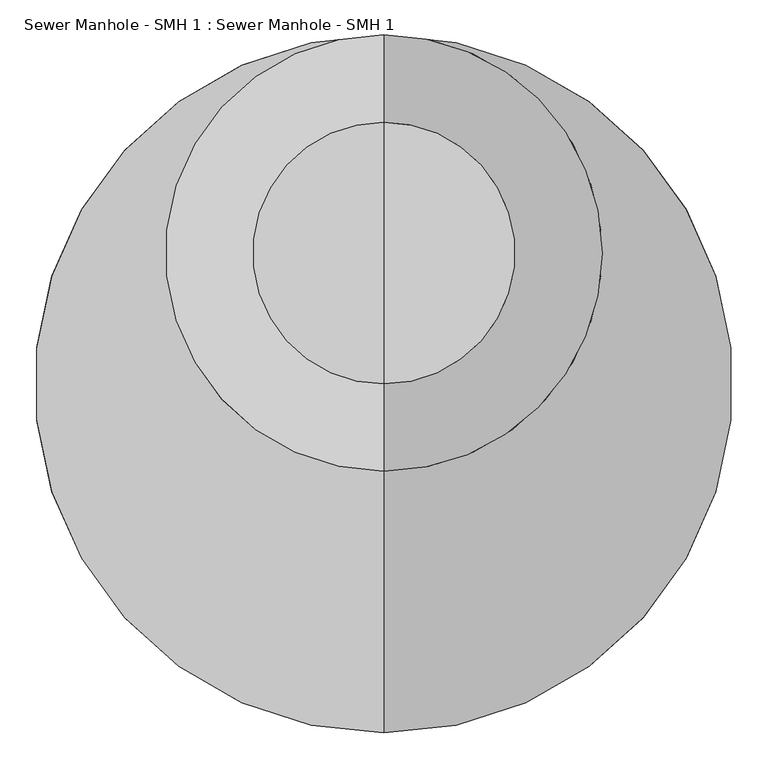
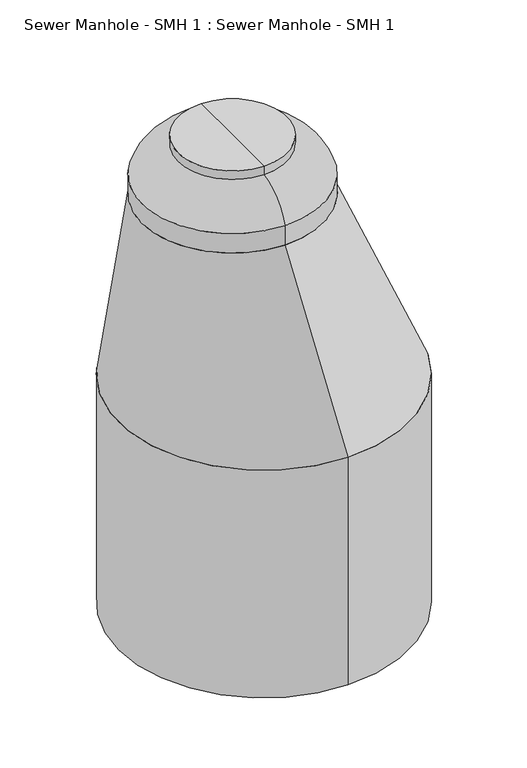
"""IFC4 building model written with IfcOpenShell, lengths in millimetres: proxy geometry, Sewer Manhole - SMH 1 : Sewer Manhole - SMH 1."""

from ifc_helpers import new_model, si_unit, point, frame, origin, place, context, project, spatial, circle_curve, ellipse_curve, trimmed, source, transform, mapped, element, save
from ifc_brep_helpers import plane_surface, cylinder_surface, revolved_surface, spline_surface, advanced_brep


def sewer_manhole_smh_1_sewer_manhole_smh_1_fd977433(model_context):
    return source(origin(), model_context, "Body", "AdvancedBrep", [
        advanced_brep(
        [(0.0, 812.8, 2231.8870774), (0.0, -203.2, 2231.8870774), (0.0, 812.8, 1346.2), (0.0, -812.8, 1346.2)],
        [
            (0, 1, circle_curve(frame((0.0, 304.8, 2231.8870774), z_axis=(0.0, 0.0, 1.0), x_axis=(0.0, 1.0, 0.0)), 508.0)),
            (1, 0, circle_curve(frame((0.0, 304.8, 2231.8870774), z_axis=(0.0, 0.0, 1.0), x_axis=(0.0, 1.0, 0.0)), 508.0)),
            (2, 3, circle_curve(frame((0.0, 0.0, 1346.2), z_axis=(0.0, 0.0, -1.0), x_axis=(0.0, 1.0, 0.0)), 812.8)),
            (3, 2, circle_curve(frame((0.0, 0.0, 1346.2), z_axis=(0.0, 0.0, -1.0), x_axis=(0.0, 1.0, 0.0)), 812.8)),
            (3, 1),
            (0, 2),
        ],
        [
            plane_surface(frame((0.0, 304.8, 2231.8870774), z_axis=(0.0, 0.0, 1.0), x_axis=(1.0, 0.0, 0.0))),
            plane_surface(frame((0.0, 0.0, 1346.2), z_axis=(0.0, 0.0, -1.0), x_axis=(1.0, 0.0, 0.0))),
            spline_surface(2, 1, [[(0.0, 812.8, 1346.2), (0.0, 812.8, 2231.8870774)], [(-812.8, 812.8, 1346.2), (-507.99999999999994, 812.8, 2231.8870774)], [(-812.8, 0.0, 1346.2), (-507.99999999999994, 304.8, 2231.8870774)], [(-812.8, -812.8, 1346.2), (-507.99999999999994, -203.19999999999993, 2231.8870774)], [(0.0, -812.8, 1346.2), (0.0, -203.2, 2231.8870774)]], [3, 2, 3], [2, 2], [0.0, 1.0, 2.0], [0.0, 1.0], weights=[[1.0, 1.0], [0.7071067811865476, 0.7071067811865476], [1.0, 1.0], [0.7071067811865476, 0.7071067811865476], [1.0, 1.0]]),
            spline_surface(2, 1, [[(0.0, -812.8, 1346.2), (0.0, -203.2, 2231.8870774)], [(812.8, -812.8, 1346.2), (508.0, -203.2, 2231.8870774)], [(812.8, 0.0, 1346.2), (508.0, 304.8, 2231.8870774)], [(812.8, 812.8, 1346.2), (508.0, 812.8, 2231.8870774)], [(0.0, 812.8, 1346.2), (0.0, 812.8, 2231.8870774)]], [3, 2, 3], [2, 2], [0.0, 1.0, 2.0], [0.0, 1.0], weights=[[1.0, 1.0], [0.7071067811865476, 0.7071067811865476], [1.0, 1.0], [0.7071067811865476, 0.7071067811865476], [1.0, 1.0]]),
        ],
        [
            (0, [[1, 2]]),
            (1, [[3, 4]]),
            (2, [[-4, 5, -1, 6]]),
            (3, [[-3, -6, -2, -5]]),
        ],
    ),
        advanced_brep(
        [(0.0, -203.2, 2231.8870774), (0.0, 812.8, 2231.8870774), (0.0, 304.8, 2231.8870774), (0.0, -203.2, 2346.96), (0.0, 812.8, 2346.96), (0.0, 0.0, 2524.76), (0.0, 609.6, 2524.76), (0.0, 0.0, 2575.56), (0.0, 609.6, 2575.56), (0.0, 304.8, 2575.56)],
        [
            (0, 1, circle_curve(frame((0.0, 304.8, 2231.8870774), z_axis=(0.0, 0.0, -1.0), x_axis=(0.0, 1.0, 0.0)), 508.0)),
            (1, 2),
            (2, 0),
            (1, 0, circle_curve(frame((0.0, 304.8, 2231.8870774), z_axis=(0.0, 0.0, -1.0), x_axis=(0.0, 1.0, 0.0)), 508.0)),
            (3, 4, circle_curve(frame((0.0, 304.8, 2346.96), z_axis=(0.0, 0.0, -1.0), x_axis=(0.0, 1.0, 0.0)), 508.0)),
            (4, 1),
            (0, 3),
            (4, 3, circle_curve(frame((0.0, 304.8, 2346.96), z_axis=(0.0, 0.0, -1.0), x_axis=(0.0, 1.0, 0.0)), 508.0)),
            (5, 6, circle_curve(frame((0.0, 304.8, 2524.76), z_axis=(0.0, 0.0, -1.0), x_axis=(0.0, 1.0, 0.0)), 304.8)),
            (6, 4, circle_curve(frame((0.0, 564.4539436, 2268.1502213), z_axis=(-1.0, 0.0, 0.0), x_axis=(0.0, -1.0, 0.0)), 260.550849)),
            (3, 5, circle_curve(frame((0.0, 45.1460564, 2268.1502213), z_axis=(-1.0, 0.0, 0.0), x_axis=(0.0, 1.0, 0.0)), 260.550849)),
            (6, 5, circle_curve(frame((0.0, 304.8, 2524.76), z_axis=(0.0, 0.0, -1.0), x_axis=(0.0, 1.0, 0.0)), 304.8)),
            (7, 8, circle_curve(frame((0.0, 304.8, 2575.56), z_axis=(0.0, 0.0, -1.0), x_axis=(0.0, 1.0, 0.0)), 304.8)),
            (8, 6),
            (5, 7),
            (8, 7, circle_curve(frame((0.0, 304.8, 2575.56), z_axis=(0.0, 0.0, -1.0), x_axis=(0.0, 1.0, 0.0)), 304.8)),
            (9, 8),
            (7, 9),
        ],
        [
            plane_surface(frame((0.0, 304.8, 2231.8870774), z_axis=(0.0, 0.0, -1.0), x_axis=(0.0, 1.0, 0.0))),
            cylinder_surface(frame((0.0, 304.8, 2296.16), z_axis=(0.0, 0.0, 1.0), x_axis=(0.0, 1.0, 0.0)), 508.0),
            revolved_surface(trimmed(ellipse_curve(frame((0.0, 564.4539436, 2268.1502213), z_axis=(1.0, 0.0, 0.0), x_axis=(0.0, -1.0, 0.0)), 260.550849, 260.550849), [point((0.0, 812.8, 2346.96))], [point((0.0, 609.6, 2524.76))], True, "CARTESIAN"), (0.0, 304.8, 2296.16), (0.0, 0.0, 1.0)),
            cylinder_surface(frame((0.0, 304.8, 2296.16), z_axis=(0.0, 0.0, 1.0), x_axis=(0.0, 1.0, 0.0)), 304.8),
            plane_surface(frame((0.0, 304.8, 2575.56), z_axis=(0.0, 0.0, 1.0), x_axis=(0.0, 1.0, 0.0))),
        ],
        [
            (0, [[1, 2, 3]]),
            (0, [[4, -3, -2]]),
            (1, [[5, 6, -1, 7]]),
            (1, [[8, -7, -4, -6]]),
            (2, [[9, 10, -5, 11]]),
            (2, [[12, -11, -8, -10]]),
            (3, [[13, 14, -9, 15]]),
            (3, [[16, -15, -12, -14]]),
            (4, [[17, -13, 18]]),
            (4, [[-18, -16, -17]]),
        ],
    ),
        advanced_brep(
        [(0.0, -812.8, 1346.2), (0.0, 812.8, 1346.2), (0.0, 812.8, 0.0), (0.0, -812.8, 0.0), (0.0, 0.0, 0.0), (0.0, 0.0, 1346.2)],
        [
            (0, 1, circle_curve(frame((0.0, 0.0, 1346.2), z_axis=(0.0, 0.0, -1.0), x_axis=(0.0, 1.0, 0.0)), 812.8)),
            (1, 2),
            (2, 3, circle_curve(frame((0.0, 0.0, 0.0), z_axis=(0.0, 0.0, 1.0), x_axis=(0.0, 1.0, 0.0)), 812.8)),
            (3, 0),
            (1, 0, circle_curve(frame((0.0, 0.0, 1346.2), z_axis=(0.0, 0.0, -1.0), x_axis=(0.0, 1.0, 0.0)), 812.8)),
            (3, 2, circle_curve(frame((0.0, 0.0, 0.0), z_axis=(0.0, 0.0, 1.0), x_axis=(0.0, 1.0, 0.0)), 812.8)),
            (2, 4),
            (4, 3),
            (5, 1),
            (0, 5),
        ],
        [
            cylinder_surface(frame((0.0, 0.0, 457.2), z_axis=(0.0, 0.0, 1.0), x_axis=(0.0, 1.0, 0.0)), 812.8),
            plane_surface(frame((0.0, 0.0, 0.0), z_axis=(0.0, 0.0, -1.0), x_axis=(0.0, 1.0, 0.0))),
            plane_surface(frame((0.0, 0.0, 1346.2), z_axis=(0.0, 0.0, 1.0), x_axis=(0.0, 1.0, 0.0))),
        ],
        [
            (0, [[1, 2, 3, 4]]),
            (0, [[5, -4, 6, -2]]),
            (1, [[-3, 7, 8]]),
            (1, [[-6, -8, -7]]),
            (2, [[9, -1, 10]]),
            (2, [[-10, -5, -9]]),
        ],
    ),
    ])


if __name__ == "__main__":
    model = new_model("IFC4")
    model_context = context("Model", 3, world=origin())
    ifc_project = project(units=[si_unit("LENGTHUNIT", "METRE", prefix="MILLI")], contexts=[model_context])
    site = spatial("IfcSite", under=ifc_project)
    building = spatial("IfcBuilding", under=site)
    placement = place(None, origin())
    sewer_manhole_smh_1_sewer_manhole_smh_1_shape = sewer_manhole_smh_1_sewer_manhole_smh_1_fd977433(model_context)
    element("IfcBuildingElementProxy", 1, Name="Sewer Manhole - SMH 1 : Sewer Manhole - SMH 1", ObjectType="Sewer Manhole - SMH 1 : Sewer Manhole - SMH 1", at=placement, inside=building, context=model_context, shape_type="MappedRepresentation", body=[
        mapped(sewer_manhole_smh_1_sewer_manhole_smh_1_shape, transform((0.0, 0.0, 0.0), x_axis=(1.0, 0.0, 0.0), y_axis=(0.0, 1.0, 0.0), z_axis=(0.0, 0.0, 1.0))),
    ])
    save(model, "model.ifc")
